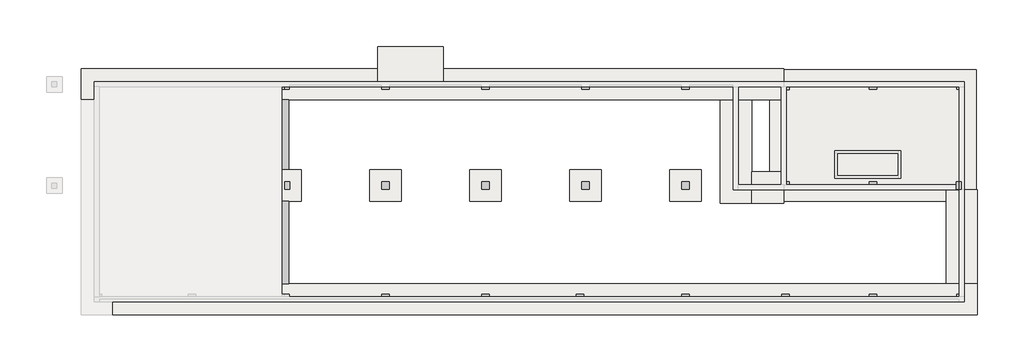
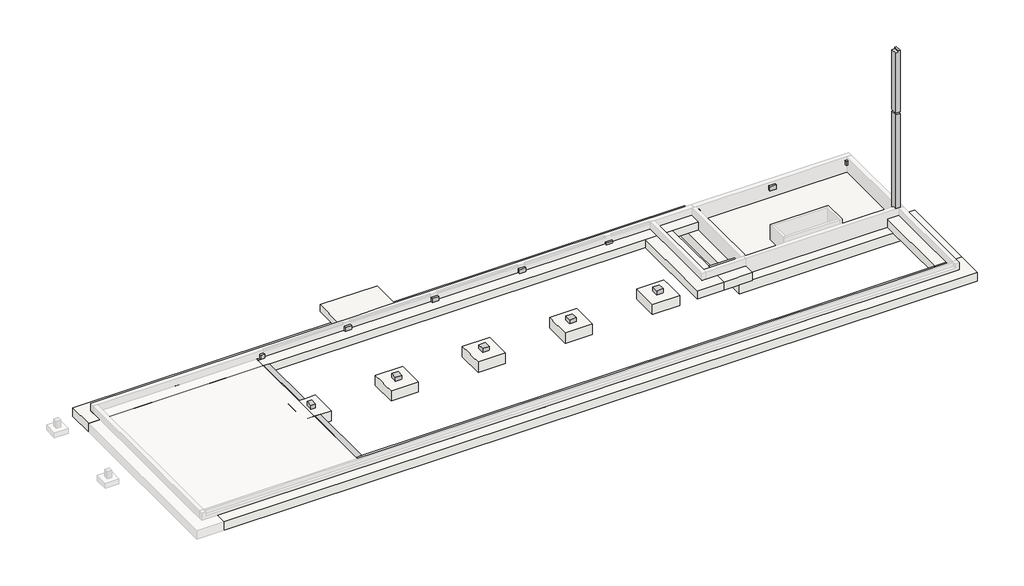
# Not in any storey, part 2 of 2: 25 columns, 8 beams, 8 slabs, 5 footings.
"""IFC4 building model written with IfcOpenShell, lengths in millimetres."""

from ifc_helpers import new_model, si_unit, frame, origin, place, context, project, spatial, polyline, outline, extrude, faceted_brep, element, save

model = new_model("IFC4")

# Units and contexts
model_context = context("Model", 3, world=origin())
ifc_project = project(units=[si_unit("LENGTHUNIT", "METRE", prefix="MILLI")], contexts=[model_context])

# Site, building
site = spatial("IfcSite", under=ifc_project)
building = spatial("IfcBuilding", under=site)

# Beams
placement = place(None, origin())
element("IfcBeam", 1, ObjectType="RC Beam_Rectangular : H_SB_AR_S16_TG_B600xH800_FG2", at=placement, inside=building, context=model_context, shape_type="Brep", body=[
    faceted_brep([(1150.0, 9199.5208589, -1350.0381366), (6250.0, 9199.5208589, -1350.0381366), (6250.0, 9199.5208589, -700.0381366), (4000.0, 9199.5208589, -700.0381366), (3500.0, 9199.5208589, -700.0381366), (1150.0, 9199.5208589, -700.0381366), (1150.0, 9799.5208589, -1350.0381366), (6250.0, 9799.5208589, -1350.0381366), (1150.0, 9799.5208589, -700.0381366), (3500.0, 9799.5208589, -700.0381366), (4000.0, 9799.5208589, -700.0381366), (6250.0, 9799.5208589, -700.0381366)], [[[0, 1, 2, 3, 4, 5]], [[0, 6, 7, 1]], [[7, 6, 8, 9, 10, 11]], [[6, 0, 5, 8]], [[1, 7, 11, 2]], [[5, 4, 3, 2, 11, 10, 9, 8]]]),
])
element("IfcBeam", 2, ObjectType="RC Beam_Rectangular : H_SB_AR_S16_TG_B600xH800_FG2", at=placement, inside=building, context=model_context, shape_type="Brep", body=[
    faceted_brep([(8750.0, 9199.5208589, -1350.0381366), (13750.0, 9199.5208589, -1350.0381366), (13750.0, 9199.5208589, -700.0381366), (11500.0, 9199.5208589, -700.0381366), (11000.0, 9199.5208589, -700.0381366), (8750.0, 9199.5208589, -700.0381366), (8750.0, 9799.5208589, -1350.0381366), (13750.0, 9799.5208589, -1350.0381366), (8750.0, 9799.5208589, -700.0381366), (11000.0, 9799.5208589, -700.0381366), (11500.0, 9799.5208589, -700.0381366), (13750.0, 9799.5208589, -700.0381366)], [[[0, 1, 2, 3, 4, 5]], [[0, 6, 7, 1]], [[7, 6, 8, 9, 10, 11]], [[6, 0, 5, 8]], [[1, 7, 11, 2]], [[5, 4, 3, 2, 11, 10, 9, 8]]]),
])
element("IfcBeam", 3, ObjectType="RC Beam_Rectangular : H_SB_AR_S16_TG_B500xH700_FB1", at=placement, inside=building, context=model_context, shape_type="SweptSolid", body=[
    extrude(outline(polyline([(4000.0, 9799.5208589), (3500.0, 9799.5208589), (3500.0, 16349.5208589), (4000.0, 16349.5208589), (4000.0, 9799.5208589)])), frame((0.0, 0.0, -1250.0381366), z_axis=(0.0, 0.0, 1.0), x_axis=(1.0, 0.0, 0.0)), (0.0, 0.0, 1.0), 550.0),
])
element("IfcBeam", 4, ObjectType="RC Beam_Rectangular : H_SB_AR_S16_TG_B500xH700_FB1", at=placement, inside=building, context=model_context, shape_type="SweptSolid", body=[
    extrude(outline(polyline([(11500.0, 9799.5208589), (11000.0, 9799.5208589), (11000.0, 16349.5208589), (11500.0, 16349.5208589), (11500.0, 9799.5208589)])), frame((0.0, 0.0, -1250.0381366), z_axis=(0.0, 0.0, 1.0), x_axis=(1.0, 0.0, 0.0)), (0.0, 0.0, 1.0), 550.0),
])
element("IfcBeam", 5, ObjectType="RC Beam_Rectangular : H_SB_AR_S16_TG_B500xH700_FB1", at=placement, inside=building, context=model_context, shape_type="SweptSolid", body=[
    extrude(outline(polyline([(11500.0, 1649.5208589), (11000.0, 1649.5208589), (11000.0, 9199.5208589), (11500.0, 9199.5208589), (11500.0, 1649.5208589)])), frame((0.0, 0.0, -1250.0381366), z_axis=(0.0, 0.0, 1.0), x_axis=(1.0, 0.0, 0.0)), (0.0, 0.0, 1.0), 550.0),
])
element("IfcBeam", 6, ObjectType="RC Beam_Rectangular : H_SB_AR_S16_TG_B500xH700_FG1", at=placement, inside=building, context=model_context, shape_type="SweptSolid", body=[
    extrude(outline(polyline([(7250.0, 16349.5208589), (7750.0, 16349.5208589), (7750.0, 10749.5208589), (7250.0, 10749.5208589), (7250.0, 16349.5208589)])), frame((0.0, 0.0, -1250.0381366), z_axis=(0.0, 0.0, 1.0), x_axis=(1.0, 0.0, 0.0)), (0.0, 0.0, 1.0), 550.0),
])
element("IfcBeam", 7, ObjectType="RC Beam_Rectangular : H_SB_AR_S16_TG_B500xH700_FG1", at=placement, inside=building, context=model_context, shape_type="SweptSolid", body=[
    extrude(outline(polyline([(14750.0, 16349.5208589), (15250.0, 16349.5208589), (15250.0, 10749.5208589), (14750.0, 10749.5208589), (14750.0, 16349.5208589)])), frame((0.0, 0.0, -1250.0381366), z_axis=(0.0, 0.0, 1.0), x_axis=(1.0, 0.0, 0.0)), (0.0, 0.0, 1.0), 700.0),
])
element("IfcBeam", 8, ObjectType="RC Beam_Rectangular : H_SB_AR_S16_TG_B500xH700_FG1", at=placement, inside=building, context=model_context, shape_type="SweptSolid", body=[
    extrude(outline(polyline([(15250.0, 1649.5208589), (14750.0, 1649.5208589), (14750.0, 8249.5208589), (15250.0, 8249.5208589), (15250.0, 1649.5208589)])), frame((0.0, 0.0, -1250.0381366), z_axis=(0.0, 0.0, 1.0), x_axis=(1.0, 0.0, 0.0)), (0.0, 0.0, 1.0), 700.0),
])

# Columns
element("IfcColumn", 9, ObjectType="RC_Column_Rectangular : H_SC_AR_S15_UG_W600xL600_C2", at=placement, inside=building, context=model_context, shape_type="Brep", body=[
    faceted_brep([(300.0, 17799.5208589, -850.0381366), (300.0, 17199.5208589, -850.0381366), (-300.0, 17199.5208589, -850.0381366), (-300.0, 17799.5208589, -850.0381366), (300.0, 17799.5208589, -550.0381366), (300.0, 17399.5208589, -550.0381366), (300.0, 17399.5208589, -700.0381366), (300.0, 17199.5208589, -700.0381366), (-300.0, 17199.5208589, -550.0381366), (-300.0, 17399.5208589, -550.0381366), (-300.0, 17799.5208589, -550.0381366), (100.0, 17199.5208589, -550.0381366), (100.0, 17399.5208589, -550.0381366), (100.0, 17399.5208589, -700.0381366), (100.0, 17199.5208589, -700.0381366)], [[[0, 1, 2, 3]], [[1, 0, 4, 5, 6, 7]], [[3, 2, 8, 9, 10]], [[0, 3, 10, 4]], [[8, 11, 12, 5, 4, 10, 9]], [[6, 13, 14, 7]], [[13, 12, 11, 14]], [[12, 13, 6, 5]], [[2, 1, 7, 14, 11, 8]]]),
])
element("IfcColumn", 10, ObjectType="RC_Column_Rectangular : H_SC_AR_S15_UG_W600xL600_C2", at=placement, inside=building, context=model_context, shape_type="SweptSolid", body=[
    extrude(outline(polyline([(17799.5208589, -850.0381366), (17199.5208589, -850.0381366), (17199.5208589, -700.0381366), (17399.5208589, -700.0381366), (17399.5208589, -550.0381366), (17799.5208589, -550.0381366), (17799.5208589, -850.0381366)])), frame((7200.0, 0.0, 0.0), z_axis=(1.0, 0.0, 0.0), x_axis=(0.0, 1.0, 0.0)), (0.0, 0.0, 1.0), 600.0),
])
element("IfcColumn", 11, ObjectType="RC_Column_Rectangular : H_SC_AR_S15_UG_W600xL600_C2", at=placement, inside=building, context=model_context, shape_type="Brep", body=[
    faceted_brep([(15300.0, 17799.5208589, -850.0381366), (15300.0, 17199.5208589, -850.0381366), (14700.0, 17199.5208589, -850.0381366), (14700.0, 17799.5208589, -850.0381366), (15300.0, 17799.5208589, -550.0381366), (15300.0, 17399.5208589, -550.0381366), (15300.0, 17399.5208589, -150.0381366), (15300.0, 17199.5208589, -150.0381366), (14950.0, 17199.5208589, -150.0381366), (14950.0, 17199.5208589, -550.0381366), (14700.0, 17199.5208589, -550.0381366), (14700.0, 17399.5208589, -550.0381366), (14700.0, 17799.5208589, -550.0381366), (14950.0, 17399.5208589, -150.0381366), (14950.0, 17399.5208589, -550.0381366)], [[[0, 1, 2, 3]], [[1, 0, 4, 5, 6, 7]], [[2, 1, 7, 8, 9, 10]], [[3, 2, 10, 11, 12]], [[0, 3, 12, 4]], [[8, 7, 6, 13]], [[14, 9, 8, 13]], [[9, 14, 5, 4, 12, 11, 10]], [[5, 14, 13, 6]]]),
])
element("IfcColumn", 12, ObjectType="RC_Column_Rectangular : H_SC_AR_S15_UG_W600xL600_C2", at=placement, inside=building, context=model_context, shape_type="SweptSolid", body=[
    extrude(outline(polyline([(17799.5208589, -850.0381366), (17199.5208589, -850.0381366), (17199.5208589, -150.0381366), (17399.5208589, -150.0381366), (17399.5208589, -550.0381366), (17799.5208589, -550.0381366), (17799.5208589, -850.0381366)])), frame((22700.0, 0.0, 0.0), z_axis=(1.0, 0.0, 0.0), x_axis=(0.0, 1.0, 0.0)), (0.0, 0.0, 1.0), 600.0),
])
element("IfcColumn", 13, ObjectType="RC_Column_Rectangular : H_SC_AR_S15_UG_W600xL600_C2", at=placement, inside=building, context=model_context, shape_type="SweptSolid", body=[
    extrude(outline(polyline([(17799.5208589, -850.0381366), (17199.5208589, -850.0381366), (17199.5208589, -150.0381366), (17399.5208589, -150.0381366), (17399.5208589, -550.0381366), (17799.5208589, -550.0381366), (17799.5208589, -850.0381366)])), frame((30700.0, 0.0, 0.0), z_axis=(1.0, 0.0, 0.0), x_axis=(0.0, 1.0, 0.0)), (0.0, 0.0, 1.0), 600.0),
])
element("IfcColumn", 14, ObjectType="RC_Column_Rectangular : H_SC_AR_S15_UG_W600xL600_C2", at=placement, inside=building, context=model_context, shape_type="SweptSolid", body=[
    extrude(outline(polyline([(17799.5208589, -850.0381366), (17199.5208589, -850.0381366), (17199.5208589, -150.0381366), (17399.5208589, -150.0381366), (17399.5208589, -550.0381366), (17799.5208589, -550.0381366), (17799.5208589, -850.0381366)])), frame((38700.0, 0.0, 0.0), z_axis=(1.0, 0.0, 0.0), x_axis=(0.0, 1.0, 0.0)), (0.0, 0.0, 1.0), 600.0),
])
element("IfcColumn", 15, ObjectType="RC_Column_Rectangular : H_SC_AR_S15_UG_W600xL600_C2", at=placement, inside=building, context=model_context, shape_type="SweptSolid", body=[
    extrude(outline(polyline([(17799.5208589, -850.0381366), (17199.5208589, -850.0381366), (17199.5208589, -359.953022), (17399.5208589, -359.953022), (17399.5208589, -550.0381366), (17799.5208589, -550.0381366), (17799.5208589, -850.0381366)])), frame((46700.0, 0.0, 0.0), z_axis=(1.0, 0.0, 0.0), x_axis=(0.0, 1.0, 0.0)), (0.0, 0.0, 1.0), 600.0),
])
element("IfcColumn", 16, ObjectType="RC_Column_Rectangular : H_SC_AR_S15_UG_W600xL600_C2", at=placement, inside=building, context=model_context, shape_type="Brep", body=[
    faceted_brep([(69300.0, 799.5208589, -850.0381366), (69300.0, 199.5208589, -850.0381366), (68700.0, 199.5208589, -850.0381366), (68700.0, 799.5208589, -850.0381366), (69300.0, 799.5208589, -550.0381366), (69300.0, 599.5208589, -550.0381366), (69300.0, 199.5208589, -550.0381366), (68700.0, 199.5208589, -550.0381366), (68700.0, 599.5208589, -550.0381366), (68700.0, 599.5208589, -150.0381366), (68700.0, 799.5208589, -150.0381366), (68900.0, 799.5208589, -150.0381366), (68900.0, 799.5208589, -550.0381366), (68900.0, 599.5208589, -150.0381366), (68900.0, 599.5208589, -550.0381366)], [[[0, 1, 2, 3]], [[1, 0, 4, 5, 6]], [[2, 1, 6, 7]], [[3, 2, 7, 8, 9, 10]], [[0, 3, 10, 11, 12, 4]], [[10, 9, 13, 11]], [[9, 8, 14, 13]], [[4, 12, 14, 8, 7, 6, 5]], [[14, 12, 11, 13]]]),
])
element("IfcColumn", 17, ObjectType="RC_Column_Rectangular : H_SC_AR_S15_UG_W600xL600_C2", at=placement, inside=building, context=model_context, shape_type="SweptSolid", body=[
    extrude(outline(polyline([(799.5208589, -850.0381366), (199.5208589, -850.0381366), (199.5208589, -550.0381366), (599.5208589, -550.0381366), (599.5208589, -150.0381366), (799.5208589, -150.0381366), (799.5208589, -850.0381366)])), frame((61700.0, 0.0, 0.0), z_axis=(1.0, 0.0, 0.0), x_axis=(0.0, 1.0, 0.0)), (0.0, 0.0, 1.0), 600.0),
])
element("IfcColumn", 18, ObjectType="RC_Column_Rectangular : H_SC_AR_S15_UG_W600xL600_C2", at=placement, inside=building, context=model_context, shape_type="SweptSolid", body=[
    extrude(outline(polyline([(799.5208589, -850.0381366), (199.5208589, -850.0381366), (199.5208589, -550.0381366), (599.5208589, -550.0381366), (599.5208589, -150.0381366), (799.5208589, -150.0381366), (799.5208589, -850.0381366)])), frame((54700.0, 0.0, 0.0), z_axis=(1.0, 0.0, 0.0), x_axis=(0.0, 1.0, 0.0)), (0.0, 0.0, 1.0), 600.0),
])
element("IfcColumn", 19, ObjectType="RC_Column_Rectangular : H_SC_AR_S15_UG_W600xL600_C2", at=placement, inside=building, context=model_context, shape_type="SweptSolid", body=[
    extrude(outline(polyline([(799.5208589, -850.0381366), (199.5208589, -850.0381366), (199.5208589, -550.0381366), (599.5208589, -550.0381366), (599.5208589, -150.0381366), (799.5208589, -150.0381366), (799.5208589, -850.0381366)])), frame((46700.0, 0.0, 0.0), z_axis=(1.0, 0.0, 0.0), x_axis=(0.0, 1.0, 0.0)), (0.0, 0.0, 1.0), 600.0),
])
element("IfcColumn", 20, ObjectType="RC_Column_Rectangular : H_SC_AR_S15_UG_W600xL600_C2", at=placement, inside=building, context=model_context, shape_type="SweptSolid", body=[
    extrude(outline(polyline([(799.5208589, -850.0381366), (199.5208589, -850.0381366), (199.5208589, -550.0381366), (599.5208589, -550.0381366), (599.5208589, -150.0381366), (799.5208589, -150.0381366), (799.5208589, -850.0381366)])), frame((38250.0, 0.0, 0.0), z_axis=(1.0, 0.0, 0.0), x_axis=(0.0, 1.0, 0.0)), (0.0, 0.0, 1.0), 600.0),
])
element("IfcColumn", 21, ObjectType="RC_Column_Rectangular : H_SC_AR_S15_UG_W600xL600_C2", at=placement, inside=building, context=model_context, shape_type="SweptSolid", body=[
    extrude(outline(polyline([(799.5208589, -850.0381366), (199.5208589, -850.0381366), (199.5208589, -550.0381366), (599.5208589, -550.0381366), (599.5208589, -150.0381366), (799.5208589, -150.0381366), (799.5208589, -850.0381366)])), frame((30700.0, 0.0, 0.0), z_axis=(1.0, 0.0, 0.0), x_axis=(0.0, 1.0, 0.0)), (0.0, 0.0, 1.0), 600.0),
])
element("IfcColumn", 22, ObjectType="RC_Column_Rectangular : H_SC_AR_S15_UG_W600xL600_C2", at=placement, inside=building, context=model_context, shape_type="SweptSolid", body=[
    extrude(outline(polyline([(799.5208589, -850.0381366), (199.5208589, -850.0381366), (199.5208589, -550.0381366), (599.5208589, -550.0381366), (599.5208589, -150.0381366), (799.5208589, -150.0381366), (799.5208589, -850.0381366)])), frame((22700.0, 0.0, 0.0), z_axis=(1.0, 0.0, 0.0), x_axis=(0.0, 1.0, 0.0)), (0.0, 0.0, 1.0), 600.0),
])
element("IfcColumn", 23, ObjectType="RC_Column_Rectangular : H_SC_AR_S15_AG_W600xL600_C2", at=placement, inside=building, context=model_context, shape_type="SweptSolid", body=[
    extrude(outline(polyline([(15350.0, 9799.5208589), (15350.0, 9199.5208589), (14950.0, 9199.5208589), (14950.0, 9799.5208589), (15350.0, 9799.5208589)])), frame((0.0, 0.0, -550.0381366), z_axis=(0.0, 0.0, 1.0), x_axis=(1.0, 0.0, 0.0)), (0.0, 0.0, 1.0), 400.0),
])
element("IfcColumn", 24, ObjectType="RC_Column_Rectangular : H_SC_AR_S15_AG_W600xL600_C2", at=placement, inside=building, context=model_context, shape_type="SweptSolid", body=[
    extrude(outline(polyline([(23300.0, 9799.5208589), (23300.0, 9199.5208589), (22700.0, 9199.5208589), (22700.0, 9799.5208589), (23300.0, 9799.5208589)])), frame((0.0, 0.0, -550.0381366), z_axis=(0.0, 0.0, 1.0), x_axis=(1.0, 0.0, 0.0)), (0.0, 0.0, 1.0), 400.0),
])
element("IfcColumn", 25, ObjectType="RC_Column_Rectangular : H_SC_AR_S15_AG_W600xL600_C2", at=placement, inside=building, context=model_context, shape_type="SweptSolid", body=[
    extrude(outline(polyline([(31300.0, 9799.5208589), (31300.0, 9199.5208589), (30700.0, 9199.5208589), (30700.0, 9799.5208589), (31300.0, 9799.5208589)])), frame((0.0, 0.0, -550.0381366), z_axis=(0.0, 0.0, 1.0), x_axis=(1.0, 0.0, 0.0)), (0.0, 0.0, 1.0), 400.0),
])
element("IfcColumn", 26, ObjectType="RC_Column_Rectangular : H_SC_AR_S15_AG_W600xL600_C2", at=placement, inside=building, context=model_context, shape_type="SweptSolid", body=[
    extrude(outline(polyline([(39300.0, 9799.5208589), (39300.0, 9199.5208589), (38700.0, 9199.5208589), (38700.0, 9799.5208589), (39300.0, 9799.5208589)])), frame((0.0, 0.0, -550.0381366), z_axis=(0.0, 0.0, 1.0), x_axis=(1.0, 0.0, 0.0)), (0.0, 0.0, 1.0), 400.0),
])
element("IfcColumn", 27, ObjectType="RC_Column_Rectangular : H_SC_AR_S15_AG_W600xL600_C2", at=placement, inside=building, context=model_context, shape_type="SweptSolid", body=[
    extrude(outline(polyline([(47300.0, 9799.5208589), (47300.0, 9199.5208589), (46700.0, 9199.5208589), (46700.0, 9799.5208589), (47300.0, 9799.5208589)])), frame((0.0, 0.0, -550.0381366), z_axis=(0.0, 0.0, 1.0), x_axis=(1.0, 0.0, 0.0)), (0.0, 0.0, 1.0), 400.0),
])
element("IfcColumn", 28, ObjectType="RC_Column_Rectangular : H_SC_AR_S15_AG_W600xL600_C2", at=placement, inside=building, context=model_context, shape_type="SweptSolid", body=[
    extrude(outline(polyline([(55300.0, 9799.5208589), (55300.0, 9549.5208589), (55050.0, 9549.5208589), (55050.0, 9799.5208589), (55300.0, 9799.5208589)])), frame((0.0, 0.0, -550.0381366), z_axis=(0.0, 0.0, 1.0), x_axis=(1.0, 0.0, 0.0)), (0.0, 0.0, 1.0), 400.0),
])
element("IfcColumn", 29, ObjectType="RC_Column_Rectangular : H_SC_AR_S15_AG_W600xL600_C2", at=placement, inside=building, context=model_context, shape_type="SweptSolid", body=[
    extrude(outline(polyline([(61700.0, 9799.5208589), (62300.0, 9799.5208589), (62300.0, 9549.5208589), (61700.0, 9549.5208589), (61700.0, 9799.5208589)])), frame((0.0, 0.0, -550.0381366), z_axis=(0.0, 0.0, 1.0), x_axis=(1.0, 0.0, 0.0)), (0.0, 0.0, 1.0), 400.0),
])
element("IfcColumn", 30, ObjectType="RC_Column_Rectangular : H_SC_AR_S15_AG_W600xL600_C2", at=placement, inside=building, context=model_context, shape_type="Brep", body=[
    faceted_brep([(68650.0, 9799.5208589, -550.0381366), (68900.0, 9799.5208589, -550.0381366), (68900.0, 9549.5208589, -550.0381366), (68650.0, 9549.5208589, -550.0381366), (68900.0, 9799.5208589, 149.9618634), (68900.0, 9549.5208589, 149.9618634), (68650.0, 9549.5208589, 149.9618634), (69050.0, 9799.5208589, 149.9618634), (69050.0, 9199.5208589, 149.9618634), (68650.0, 9199.5208589, 149.9618634), (69050.0, 9799.5208589, 9269.9618634), (69050.0, 9199.5208589, 9269.9618634), (68650.0, 9199.5208589, 9269.9618634), (68650.0, 9799.5208589, 9269.9618634)], [[[0, 1, 2, 3]], [[1, 4, 5, 2]], [[6, 5, 4, 7, 8, 9]], [[5, 6, 3, 2]], [[8, 7, 10, 11]], [[12, 11, 10, 13]], [[9, 8, 11, 12]], [[0, 3, 6, 9, 12, 13]], [[1, 0, 13, 10, 7, 4]]]),
    faceted_brep([(69050.0, 9199.5208589, 9449.9618634), (69050.0, 9199.5208589, 15409.9618634), (68900.0, 9199.5208589, 15409.9618634), (68900.0, 9199.5208589, 15259.9618634), (68650.0, 9199.5208589, 15259.9618634), (68650.0, 9199.5208589, 9449.9618634), (68650.0, 9799.5208589, 9449.9618634), (68650.0, 9799.5208589, 15259.9618634), (69050.0, 9799.5208589, 15409.9618634), (69050.0, 9799.5208589, 9449.9618634), (68900.0, 9799.5208589, 15259.9618634), (68900.0, 9799.5208589, 15409.9618634)], [[[0, 1, 2, 3, 4, 5]], [[6, 5, 4, 7]], [[8, 9, 6, 7, 10, 11]], [[1, 8, 11, 2]], [[0, 5, 6, 9]], [[8, 1, 0, 9]], [[3, 10, 7, 4]], [[10, 3, 2, 11]]]),
])
element("IfcColumn", 31, ObjectType="RC_Column_Rectangular : H_SC_AR_S15_UG_W600xL600_C2", at=placement, inside=building, context=model_context, shape_type="SweptSolid", body=[
    extrude(outline(polyline([(68700.0, 17199.5208589), (68700.0, 17399.5208589), (68900.0, 17399.5208589), (68900.0, 17199.5208589), (68700.0, 17199.5208589)])), frame((0.0, 0.0, -550.0381366), z_axis=(0.0, 0.0, 1.0), x_axis=(1.0, 0.0, 0.0)), (0.0, 0.0, 1.0), 400.0),
])
element("IfcColumn", 32, ObjectType="RC_Column_Rectangular : H_SC_AR_S15_UG_W600xL600_C2", at=placement, inside=building, context=model_context, shape_type="SweptSolid", body=[
    extrude(outline(polyline([(62300.0, 17199.5208589), (61700.0, 17199.5208589), (61700.0, 17399.5208589), (62300.0, 17399.5208589), (62300.0, 17199.5208589)])), frame((0.0, 0.0, -550.0381366), z_axis=(0.0, 0.0, 1.0), x_axis=(1.0, 0.0, 0.0)), (0.0, 0.0, 1.0), 400.0),
])
element("IfcColumn", 33, ObjectType="RC_Column_Rectangular : H_SC_AR_S15_AG_W600xL600_C2", at=placement, inside=building, context=model_context, shape_type="SweptSolid", body=[
    extrude(outline(polyline([(54850.0, 17749.5208589), (54850.0, 17399.5208589), (54700.0, 17399.5208589), (54700.0, 17749.5208589), (54850.0, 17749.5208589)])), frame((0.0, 0.0, -550.0381366), z_axis=(0.0, 0.0, 1.0), x_axis=(1.0, 0.0, 0.0)), (0.0, 0.0, 1.0), 400.0),
    extrude(outline(polyline([(55300.0, 17399.5208589), (55300.0, 17149.5208589), (55050.0, 17149.5208589), (55050.0, 17399.5208589), (55300.0, 17399.5208589)])), frame((0.0, 0.0, -550.0381366), z_axis=(0.0, 0.0, 1.0), x_axis=(1.0, 0.0, 0.0)), (0.0, 0.0, 1.0), 400.0),
])

# Footings
element("IfcFooting", 34, ObjectType="H_SF_AR_S18_Wall FDN_T800", at=placement, inside=building, context=model_context, shape_type="Brep", body=[
    faceted_brep([(54850.0, 18849.5208589, -550.0381366), (54850.0, 16349.5208589, -550.0381366), (54850.0, 16349.5208589, -1350.0381366), (54850.0, 18849.5208589, -1350.0381366), (-1350.0, 16349.5208589, -550.0381366), (1150.0, 16349.5208589, -550.0381366), (14750.0, 16349.5208589, -550.0381366), (15250.0, 16349.5208589, -550.0381366), (49775.0, 16349.5208589, -550.0381366), (52275.0, 16349.5208589, -550.0381366), (-1350.0, 18849.5208589, -550.0381366), (-1350.0, 18849.5208589, -1350.0381366), (-1350.0, 16349.5208589, -1350.0381366), (52275.0, 16349.5208589, -1350.0381366), (49775.0, 16349.5208589, -1350.0381366), (1150.0, 16349.5208589, -1350.0381366)], [[[0, 1, 2, 3]], [[4, 5, 6, 7, 8, 9, 1, 0, 10]], [[11, 10, 0, 3]], [[12, 11, 3, 2, 13, 14, 15]], [[4, 12, 15, 14, 13, 2, 1, 9, 8, 7, 6, 5]], [[4, 10, 11, 12]]]),
])
element("IfcFooting", 35, ObjectType="H_SF_AR_S18_Wall FDN_T800", at=placement, inside=building, context=model_context, shape_type="Brep", body=[
    faceted_brep([(70350.0, -850.4791411, -550.0381366), (70350.0, 1649.5208589, -550.0381366), (67850.0, 1649.5208589, -550.0381366), (15250.0, 1649.5208589, -550.0381366), (14750.0, 1649.5208589, -550.0381366), (1150.0, 1649.5208589, -550.0381366), (1150.0, -850.4791411, -550.0381366), (70350.0, -850.4791411, -1350.0381366), (1150.0, -850.4791411, -1350.0381366), (70350.0, 1649.5208589, -1350.0381366), (1150.0, 1649.5208589, -1350.0381366), (67850.0, 1649.5208589, -1350.0381366)], [[[0, 1, 2, 3, 4, 5, 6]], [[7, 0, 6, 8]], [[9, 7, 8, 10, 11]], [[1, 9, 11, 10, 5, 4, 3, 2]], [[1, 0, 7, 9]], [[6, 5, 10, 8]]]),
])
element("IfcFooting", 36, ObjectType="H_SF_AR_S18_Wall FDN_T800", at=placement, inside=building, context=model_context, shape_type="SweptSolid", body=[
    extrude(outline(polyline([(67850.0, 9149.5208589), (70350.0, 9149.5208589), (70350.0, 1649.5208589), (67850.0, 1649.5208589), (67850.0, 9149.5208589)])), frame((0.0, 0.0, -1350.0381366), z_axis=(0.0, 0.0, 1.0), x_axis=(1.0, 0.0, 0.0)), (0.0, 0.0, 1.0), 800.0),
])
element("IfcFooting", 37, ObjectType="H_SF_AR_S18_Wall FDN_T800", at=placement, inside=building, context=model_context, shape_type="Brep", body=[
    faceted_brep([(49775.0, 16349.5208589, -550.0381366), (49775.0, 9799.5208589, -550.0381366), (49775.0, 9199.5208589, -550.0381366), (49775.0, 8099.5208589, -550.0381366), (52275.0, 8099.5208589, -550.0381366), (52275.0, 10599.5208589, -550.0381366), (52275.0, 16349.5208589, -550.0381366), (52275.0, 16349.5208589, -1350.0381366), (52275.0, 8099.5208589, -1350.0381366), (52275.0, 10599.5208589, -1350.0381366), (49775.0, 16349.5208589, -1350.0381366), (49775.0, 8099.5208589, -1350.0381366)], [[[0, 1, 2, 3, 4, 5, 6]], [[7, 6, 5, 4, 8, 9]], [[10, 7, 9, 8, 11]], [[0, 10, 11, 3, 2, 1]], [[0, 6, 7, 10]], [[4, 3, 11, 8]]]),
])
element("IfcFooting", 38, ObjectType="H_SF_AR_S18_Wall FDN_T800", at=placement, inside=building, context=model_context, shape_type="SweptSolid", body=[
    extrude(outline(polyline([(54850.0, 10599.5208589), (54850.0, 8099.5208589), (52275.0, 8099.5208589), (52275.0, 10599.5208589), (54850.0, 10599.5208589)])), frame((0.0, 0.0, -1350.0381366), z_axis=(0.0, 0.0, 1.0), x_axis=(1.0, 0.0, 0.0)), (0.0, 0.0, 1.0), 800.0),
])

# Slabs
element("IfcSlab", 39, ObjectType="H_SF_AR_B01_MAT_Bitumen_MF1", at=placement, inside=building, context=model_context, shape_type="SweptSolid", body=[
    extrude(outline(polyline([(70250.0, 18749.5208589), (70250.0, 8249.5208589), (53750.0, 8249.5208589), (53750.0, 18749.5208589), (70250.0, 18749.5208589)])), frame((0.0, 0.0, -2350.0381366), z_axis=(0.0, 0.0, 1.0), x_axis=(1.0, 0.0, 0.0)), (0.0, 0.0, 1.0), 1000.0),
])
element("IfcSlab", 40, ObjectType="H_SF_AR_B01_MAT_Bitumen_MF2", at=placement, inside=building, context=model_context, shape_type="Brep", body=[
    faceted_brep([(27625.0, 20624.5208589, -550.0381366), (27625.0, 17799.5208589, -550.0381366), (22375.0, 17799.5208589, -550.0381366), (22375.0, 20624.5208589, -550.0381366), (27625.0, 20624.5208589, 99.9618634), (22375.0, 20624.5208589, 99.9618634), (22375.0, 17799.5208589, 99.9618634), (27625.0, 17799.5208589, 99.9618634), (22375.0, 17799.5208589, -50.0381366)], [[[0, 1, 2, 3]], [[4, 5, 6, 7]], [[1, 0, 4, 7]], [[2, 1, 7, 6, 8]], [[3, 2, 8, 6, 5]], [[0, 3, 5, 4]]]),
])
element("IfcSlab", 41, ObjectType="Foundation Rectangular (Non-Pile) : H_SF_AR_S18_W2500xL2500xT1000_Bitumen_F1", at=placement, inside=building, context=model_context, shape_type="Brep", body=[
    faceted_brep([(8750.0, 10749.5208589, -1550.0381366), (8750.0, 8249.5208589, -1550.0381366), (6250.0, 8249.5208589, -1550.0381366), (6250.0, 10749.5208589, -1550.0381366), (6250.0, 10749.5208589, -700.0381366), (7250.0, 10749.5208589, -700.0381366), (7750.0, 10749.5208589, -700.0381366), (8750.0, 10749.5208589, -700.0381366), (6250.0, 8249.5208589, -700.0381366), (6250.0, 9199.5208589, -700.0381366), (6250.0, 9799.5208589, -700.0381366), (8750.0, 8249.5208589, -700.0381366), (7750.0, 8249.5208589, -700.0381366), (7250.0, 8249.5208589, -700.0381366), (8750.0, 9799.5208589, -700.0381366), (8750.0, 9199.5208589, -700.0381366)], [[[0, 1, 2, 3]], [[0, 3, 4, 5, 6, 7]], [[3, 2, 8, 9, 10, 4]], [[2, 1, 11, 12, 13, 8]], [[1, 0, 7, 14, 15, 11]], [[7, 6, 5, 4, 10, 9, 8, 13, 12, 11, 15, 14]]]),
])
element("IfcSlab", 42, ObjectType="Foundation Rectangular (Non-Pile) : H_SF_AR_S18_W2500xL2500xT1000_Bitumen_F1", at=placement, inside=building, context=model_context, shape_type="Brep", body=[
    faceted_brep([(16250.0, 10749.5208589, -550.0381366), (15250.0, 10749.5208589, -550.0381366), (14750.0, 10749.5208589, -550.0381366), (13750.0, 10749.5208589, -550.0381366), (13750.0, 8249.5208589, -550.0381366), (14750.0, 8249.5208589, -550.0381366), (15250.0, 8249.5208589, -550.0381366), (16250.0, 8249.5208589, -550.0381366), (16250.0, 9149.5208589, -550.0381366), (16250.0, 9749.5208589, -550.0381366), (16250.0, 10749.5208589, -1550.0381366), (16250.0, 8249.5208589, -1550.0381366), (13750.0, 8249.5208589, -1550.0381366), (13750.0, 10749.5208589, -1550.0381366)], [[[0, 1, 2, 3, 4, 5, 6, 7, 8, 9]], [[10, 11, 12, 13]], [[3, 2, 1, 0, 10, 13]], [[4, 3, 13, 12]], [[7, 6, 5, 4, 12, 11]], [[0, 9, 8, 7, 11, 10]]]),
])
element("IfcSlab", 43, ObjectType="Foundation Rectangular (Non-Pile) : H_SF_AR_S18_W2500xL2500xT1000_Bitumen_F1", at=placement, inside=building, context=model_context, shape_type="Brep", body=[
    faceted_brep([(24250.0, 10749.5208589, -550.0381366), (21750.0, 10749.5208589, -550.0381366), (21750.0, 9749.5208589, -550.0381366), (21750.0, 9149.5208589, -550.0381366), (21750.0, 8249.5208589, -550.0381366), (24250.0, 8249.5208589, -550.0381366), (24250.0, 9149.5208589, -550.0381366), (24250.0, 9749.5208589, -550.0381366), (24250.0, 10749.5208589, -1550.0381366), (24250.0, 8249.5208589, -1550.0381366), (21750.0, 8249.5208589, -1550.0381366), (21750.0, 10749.5208589, -1550.0381366)], [[[0, 1, 2, 3, 4, 5, 6, 7]], [[8, 9, 10, 11]], [[1, 0, 8, 11]], [[4, 3, 2, 1, 11, 10]], [[5, 4, 10, 9]], [[0, 7, 6, 5, 9, 8]]]),
])
element("IfcSlab", 44, ObjectType="Foundation Rectangular (Non-Pile) : H_SF_AR_S18_W2500xL2500xT1000_Bitumen_F1", at=placement, inside=building, context=model_context, shape_type="Brep", body=[
    faceted_brep([(32250.0, 10749.5208589, -550.0381366), (29750.0, 10749.5208589, -550.0381366), (29750.0, 9749.5208589, -550.0381366), (29750.0, 9149.5208589, -550.0381366), (29750.0, 8249.5208589, -550.0381366), (32250.0, 8249.5208589, -550.0381366), (32250.0, 9149.5208589, -550.0381366), (32250.0, 9749.5208589, -550.0381366), (32250.0, 10749.5208589, -1550.0381366), (32250.0, 8249.5208589, -1550.0381366), (29750.0, 8249.5208589, -1550.0381366), (29750.0, 10749.5208589, -1550.0381366)], [[[0, 1, 2, 3, 4, 5, 6, 7]], [[8, 9, 10, 11]], [[1, 0, 8, 11]], [[4, 3, 2, 1, 11, 10]], [[5, 4, 10, 9]], [[0, 7, 6, 5, 9, 8]]]),
])
element("IfcSlab", 45, ObjectType="Foundation Rectangular (Non-Pile) : H_SF_AR_S18_W2500xL2500xT1000_Bitumen_F1", at=placement, inside=building, context=model_context, shape_type="Brep", body=[
    faceted_brep([(40250.0, 10749.5208589, -550.0381366), (37750.0, 10749.5208589, -550.0381366), (37750.0, 9749.5208589, -550.0381366), (37750.0, 9149.5208589, -550.0381366), (37750.0, 8249.5208589, -550.0381366), (40250.0, 8249.5208589, -550.0381366), (40250.0, 9149.5208589, -550.0381366), (40250.0, 9749.5208589, -550.0381366), (40250.0, 10749.5208589, -1550.0381366), (40250.0, 8249.5208589, -1550.0381366), (37750.0, 8249.5208589, -1550.0381366), (37750.0, 10749.5208589, -1550.0381366)], [[[0, 1, 2, 3, 4, 5, 6, 7]], [[8, 9, 10, 11]], [[1, 0, 8, 11]], [[4, 3, 2, 1, 11, 10]], [[5, 4, 10, 9]], [[0, 7, 6, 5, 9, 8]]]),
])
element("IfcSlab", 46, ObjectType="Foundation Rectangular (Non-Pile) : H_SF_AR_S18_W2500xL2500xT1000_Bitumen_F1", at=placement, inside=building, context=model_context, shape_type="Brep", body=[
    faceted_brep([(48250.0, 10749.5208589, -550.0381366), (45750.0, 10749.5208589, -550.0381366), (45750.0, 9749.5208589, -550.0381366), (45750.0, 9149.5208589, -550.0381366), (45750.0, 8249.5208589, -550.0381366), (48250.0, 8249.5208589, -550.0381366), (48250.0, 9199.5208589, -550.0381366), (48250.0, 9799.5208589, -550.0381366), (48250.0, 10749.5208589, -1550.0381366), (48250.0, 8249.5208589, -1550.0381366), (45750.0, 8249.5208589, -1550.0381366), (45750.0, 10749.5208589, -1550.0381366)], [[[0, 1, 2, 3, 4, 5, 6, 7]], [[8, 9, 10, 11]], [[1, 0, 8, 11]], [[4, 3, 2, 1, 11, 10]], [[5, 4, 10, 9]], [[0, 7, 6, 5, 9, 8]]]),
])

save(model, "model.ifc")

# Revit data of these elements
# Type "RC Beam_Rectangular : H_SB_AR_S16_TG_B600xH800_FG2"
#   Type Comments = "CV-UG"
#   Type Mark = "FG2"
#   H_Q'ty Cal Type Tag = "SB-Q1A"
#   H_WM Code_1 = "A03AF032-00022 |  | M3 | Concrete Work | Superstructure Work | Structural Concrete | Cement Type-1 | 25MPa ≤ F'c (Cylinder Strength) < 30MPa |  |  |  |  | A03AF032-00022 Concrete Work Superstructure Work Structural Concrete  Cement Type-1 25MPa ≤ F'c (Cylinder Strength) < 30MPa      |  F'c (Cylinder Strength) = 24MPa"
#   H_WM Code_2 = "A03AD037-00002 |  | TON | Concrete Work | Substructure Work | Rebar Work | Deformed Bar (Non-Coat.) | 400MPa<Fy≤470MPa |  |  |  |  | A03AD037-00002 Concrete Work Substructure Work Rebar Work Deformed Bar (Non-Coat.)  400MPa<Fy≤470MPa      | ASTM A615 GRADE 60 (Fy=420MPa)"
#   H_WM Code_3 = "A03AD035-00001 |  | M2 | Concrete Work | Substructure Work | Form Work (3 times in use) | Flat Form | Dressed Lumber, Plywood or Steel Form(Wood Planks are not Allowed) incl. Chamfer |  |  |  | A03AD035-00001 Concrete Work Substructure Work Form Work (3 times in use) Flat Form     Dressed Lumber, Plywood or Steel Form(Wood Planks are not Allowed) incl. Chamfer   | Dressed Lumber, Plywood or Steel Form(Wood Planks are not Allowed) incl. Chamfer"
#   H_WM Code_4 = "A03AH056-00001 |  | M2 | Concrete Work | Concrete Protective Coating (U/G) | Bitumen/Bituminous/Asphalt Coating |  |  | A03AH056-00001 Concrete Work Concrete Protective Coating (U/G) Bitumen/Bituminous/Asphalt Coating         | Bitumen/Bituminous/Asphalt Coating"
#   H_WM Code_5 = "A03AD047-00004 |  | M2 | Concrete Work | Substructure Work | Insulation under Ground Floor | Extruded Polystyrene Insulation Board |  | 100mm≤THK | THK=(  )mm |  | A03AD047-00004 Concrete Work Substructure Work Insulation under Ground Floor Extruded Polystyrene Insulation Board       100mm≤THK | Bitumen/Bituminous/Asphalt Coating"
#   H_WM Code_6 = "A01ZZ001-00012 |  | M3 | Earth Work | - | Excavation | Soil, Mech. |  | Manual Excavation Above GWL |  |  |  | A01ZZ001-00012 Earth Work - Excavation Soil, Mech.      Manual Excavation Above GWL  | Above GWL"
#   H_WM Code_7 = "A01ZZ001-00013 |  | M3 | Earth Work | - | Excavation | Soil, Mech. |  | Manual Excavation Below GWL |  |  |  | A01ZZ001-00013 Earth Work - Excavation Soil, Mech.      Manual Excavation Below GWL  | Below GWL"
#   H_WM Code_8 = "A01ZZ003-00001 |  | M3 | Earth Work | - | Backfill | Re-use, Soil |  |  |  | Compaction=(  )% |  | A01ZZ003-00001 Earth Work - Backfill Re-use, Soil        | Compaction=( 95 )%"
#   H_WM Code_9 = "A01ZZ004-00001 |  | M3 | Earth Work | - | Disposal | Soil |  |  |  | Disposal Distance=Appx. (  )km from Site |  | A01ZZ004-00001 Earth Work - Disposal Soil        | Disposal Distance=Appx. (20 )km from Site"
#   H_WM Code_10 = "A03AH056-00001 |  | M2 | Concrete Work | Concrete Protective Coating (U/G) | Bitumen/Bituminous/Asphalt Coating |  |  | A03AH056-00001 Concrete Work Concrete Protective Coating (U/G) Bitumen/Bituminous/Asphalt Coating         | *기초바닥 Protection 은 Lean에 적용"
#   중앙부 하부근 = ""
#   중앙부 상부근 = ""
#   중앙부 보조근 = ""
#   중앙부 늑근 = ""
#   외단부 하부근 = ""
#   외단부 상부근 = ""
#   외단부 보조근 = ""
#   외단부 늑근 = ""
#   부호 = "TG2"
#   내단부 하부근 = ""
#   내단부 상부근 = ""
#   내단부 보조근 = ""
#   내단부 늑근 = ""
#   ALL 하부근 = "3-D20"
#   ALL 상부근 = "4-D20"
#   ALL 보조근 = ""
#   ALL 늑근 = "2-D10 @120"
#   H_Rebar ratio = 0.14
#   Width = 600 mm
#   Height = 800 mm
#   Length [instance default] = 1524 mm
#   b = 600 mm
#   h = 800 mm
#   hec_material3 [instance default] = none
#   hec_material2 [instance default] = none
#   hec_material1 [instance default] = none
#   Structural Material [instance default] = none
#   Assembly Code = ""
# Type "RC Beam_Rectangular : H_SB_AR_S16_TG_B500xH700_FB1"
#   Type Comments = "CV-UG"
#   Type Mark = "FB1"
#   H_Q'ty Cal Type Tag = "SB-Q1A"
#   H_WM Code_1 = "A03AF032-00022 |  | M3 | Concrete Work | Superstructure Work | Structural Concrete | Cement Type-1 | 25MPa ≤ F'c (Cylinder Strength) < 30MPa |  |  |  |  | A03AF032-00022 Concrete Work Superstructure Work Structural Concrete  Cement Type-1 25MPa ≤ F'c (Cylinder Strength) < 30MPa      |  F'c (Cylinder Strength) = 24MPa"
#   H_WM Code_2 = "A03AD037-00002 |  | TON | Concrete Work | Substructure Work | Rebar Work | Deformed Bar (Non-Coat.) | 400MPa<Fy≤470MPa |  |  |  |  | A03AD037-00002 Concrete Work Substructure Work Rebar Work Deformed Bar (Non-Coat.)  400MPa<Fy≤470MPa      | ASTM A615 GRADE 60 (Fy=420MPa)"
#   H_WM Code_3 = "A03AD035-00001 |  | M2 | Concrete Work | Substructure Work | Form Work (3 times in use) | Flat Form | Dressed Lumber, Plywood or Steel Form(Wood Planks are not Allowed) incl. Chamfer |  |  |  | A03AD035-00001 Concrete Work Substructure Work Form Work (3 times in use) Flat Form     Dressed Lumber, Plywood or Steel Form(Wood Planks are not Allowed) incl. Chamfer   | Dressed Lumber, Plywood or Steel Form(Wood Planks are not Allowed) incl. Chamfer"
#   H_WM Code_4 = "A03AH056-00001 |  | M2 | Concrete Work | Concrete Protective Coating (U/G) | Bitumen/Bituminous/Asphalt Coating |  |  | A03AH056-00001 Concrete Work Concrete Protective Coating (U/G) Bitumen/Bituminous/Asphalt Coating         | Bitumen/Bituminous/Asphalt Coating"
#   H_WM Code_5 = "A03AD047-00004 |  | M2 | Concrete Work | Substructure Work | Insulation under Ground Floor | Extruded Polystyrene Insulation Board |  | 100mm≤THK | THK=(  )mm |  | A03AD047-00004 Concrete Work Substructure Work Insulation under Ground Floor Extruded Polystyrene Insulation Board       100mm≤THK | Bitumen/Bituminous/Asphalt Coating"
#   H_WM Code_6 = "A01ZZ001-00012 |  | M3 | Earth Work | - | Excavation | Soil, Mech. |  | Manual Excavation Above GWL |  |  |  | A01ZZ001-00012 Earth Work - Excavation Soil, Mech.      Manual Excavation Above GWL  | Above GWL"
#   H_WM Code_7 = "A01ZZ001-00013 |  | M3 | Earth Work | - | Excavation | Soil, Mech. |  | Manual Excavation Below GWL |  |  |  | A01ZZ001-00013 Earth Work - Excavation Soil, Mech.      Manual Excavation Below GWL  | Below GWL"
#   H_WM Code_8 = "A01ZZ003-00001 |  | M3 | Earth Work | - | Backfill | Re-use, Soil |  |  |  | Compaction=(  )% |  | A01ZZ003-00001 Earth Work - Backfill Re-use, Soil        | Compaction=( 95 )%"
#   H_WM Code_9 = "A01ZZ004-00001 |  | M3 | Earth Work | - | Disposal | Soil |  |  |  | Disposal Distance=Appx. (  )km from Site |  | A01ZZ004-00001 Earth Work - Disposal Soil        | Disposal Distance=Appx. (20 )km from Site"
#   H_WM Code_10 = "A03AH056-00001 |  | M2 | Concrete Work | Concrete Protective Coating (U/G) | Bitumen/Bituminous/Asphalt Coating |  |  | A03AH056-00001 Concrete Work Concrete Protective Coating (U/G) Bitumen/Bituminous/Asphalt Coating         | *기초바닥 Protection 은 Lean에 적용"
#   중앙부 하부근 = ""
#   중앙부 상부근 = ""
#   중앙부 보조근 = ""
#   중앙부 늑근 = ""
#   외단부 하부근 = ""
#   외단부 상부근 = ""
#   외단부 보조근 = ""
#   외단부 늑근 = ""
#   부호 = "TG2"
#   내단부 하부근 = ""
#   내단부 상부근 = ""
#   내단부 보조근 = ""
#   내단부 늑근 = ""
#   ALL 하부근 = "3-D20"
#   ALL 상부근 = "4-D20"
#   ALL 보조근 = ""
#   ALL 늑근 = "2-D10 @120"
#   H_Rebar ratio = 0.14
#   Width = 500 mm
#   Height = 700 mm
#   Length [instance default] = 1524 mm
#   b = 500 mm
#   h = 700 mm
#   hec_material3 [instance default] = none
#   hec_material2 [instance default] = none
#   hec_material1 [instance default] = none
#   Structural Material [instance default] = none
#   Assembly Code = ""
# Type "RC Beam_Rectangular : H_SB_AR_S16_TG_B500xH700_FG1"
#   Type Comments = "CV-UG"
#   Type Mark = "FG1"
#   H_Q'ty Cal Type Tag = "SB-Q1A"
#   H_WM Code_1 = "A03AF032-00022 |  | M3 | Concrete Work | Superstructure Work | Structural Concrete | Cement Type-1 | 25MPa ≤ F'c (Cylinder Strength) < 30MPa |  |  |  |  | A03AF032-00022 Concrete Work Superstructure Work Structural Concrete  Cement Type-1 25MPa ≤ F'c (Cylinder Strength) < 30MPa      |  F'c (Cylinder Strength) = 24MPa"
#   H_WM Code_2 = "A03AD037-00002 |  | TON | Concrete Work | Substructure Work | Rebar Work | Deformed Bar (Non-Coat.) | 400MPa<Fy≤470MPa |  |  |  |  | A03AD037-00002 Concrete Work Substructure Work Rebar Work Deformed Bar (Non-Coat.)  400MPa<Fy≤470MPa      | ASTM A615 GRADE 60 (Fy=420MPa)"
#   H_WM Code_3 = "A03AD035-00001 |  | M2 | Concrete Work | Substructure Work | Form Work (3 times in use) | Flat Form | Dressed Lumber, Plywood or Steel Form(Wood Planks are not Allowed) incl. Chamfer |  |  |  | A03AD035-00001 Concrete Work Substructure Work Form Work (3 times in use) Flat Form     Dressed Lumber, Plywood or Steel Form(Wood Planks are not Allowed) incl. Chamfer   | Dressed Lumber, Plywood or Steel Form(Wood Planks are not Allowed) incl. Chamfer"
#   H_WM Code_4 = "A03AH056-00001 |  | M2 | Concrete Work | Concrete Protective Coating (U/G) | Bitumen/Bituminous/Asphalt Coating |  |  | A03AH056-00001 Concrete Work Concrete Protective Coating (U/G) Bitumen/Bituminous/Asphalt Coating         | Bitumen/Bituminous/Asphalt Coating"
#   H_WM Code_5 = "A03AD047-00004 |  | M2 | Concrete Work | Substructure Work | Insulation under Ground Floor | Extruded Polystyrene Insulation Board |  | 100mm≤THK | THK=(  )mm |  | A03AD047-00004 Concrete Work Substructure Work Insulation under Ground Floor Extruded Polystyrene Insulation Board       100mm≤THK | Bitumen/Bituminous/Asphalt Coating"
#   H_WM Code_6 = "A01ZZ001-00012 |  | M3 | Earth Work | - | Excavation | Soil, Mech. |  | Manual Excavation Above GWL |  |  |  | A01ZZ001-00012 Earth Work - Excavation Soil, Mech.      Manual Excavation Above GWL  | Above GWL"
#   H_WM Code_7 = "A01ZZ001-00013 |  | M3 | Earth Work | - | Excavation | Soil, Mech. |  | Manual Excavation Below GWL |  |  |  | A01ZZ001-00013 Earth Work - Excavation Soil, Mech.      Manual Excavation Below GWL  | Below GWL"
#   H_WM Code_8 = "A01ZZ003-00001 |  | M3 | Earth Work | - | Backfill | Re-use, Soil |  |  |  | Compaction=(  )% |  | A01ZZ003-00001 Earth Work - Backfill Re-use, Soil        | Compaction=( 95 )%"
#   H_WM Code_9 = "A01ZZ004-00001 |  | M3 | Earth Work | - | Disposal | Soil |  |  |  | Disposal Distance=Appx. (  )km from Site |  | A01ZZ004-00001 Earth Work - Disposal Soil        | Disposal Distance=Appx. (20 )km from Site"
#   H_WM Code_10 = "A03AH056-00001 |  | M2 | Concrete Work | Concrete Protective Coating (U/G) | Bitumen/Bituminous/Asphalt Coating |  |  | A03AH056-00001 Concrete Work Concrete Protective Coating (U/G) Bitumen/Bituminous/Asphalt Coating         | *기초바닥 Protection 은 Lean에 적용"
#   중앙부 하부근 = ""
#   중앙부 상부근 = ""
#   중앙부 보조근 = ""
#   중앙부 늑근 = ""
#   외단부 하부근 = ""
#   외단부 상부근 = ""
#   외단부 보조근 = ""
#   외단부 늑근 = ""
#   부호 = "TG2"
#   내단부 하부근 = ""
#   내단부 상부근 = ""
#   내단부 보조근 = ""
#   내단부 늑근 = ""
#   ALL 하부근 = "3-D20"
#   ALL 상부근 = "4-D20"
#   ALL 보조근 = ""
#   ALL 늑근 = "2-D10 @120"
#   H_Rebar ratio = 0.14
#   Width = 500 mm
#   Height = 700 mm
#   Length [instance default] = 1524 mm
#   b = 500 mm
#   h = 700 mm
#   hec_material3 [instance default] = none
#   hec_material2 [instance default] = none
#   hec_material1 [instance default] = none
#   Structural Material [instance default] = none
#   Assembly Code = ""
# Type "RC_Column_Rectangular : H_SC_AR_S15_UG_W600xL600_C2"
#   Type Comments = "CV-UG"
#   Type Mark = "C2"
#   H_Q'ty Cal Type Tag = "SB-Q1A"
#   H_WM Code_1 = "A03AF032-00022 |  | M3 | Concrete Work | Superstructure Work | Structural Concrete | Cement Type-1 | 25MPa ≤ F'c (Cylinder Strength) < 30MPa |  |  |  |  | A03AF032-00022 Concrete Work Superstructure Work Structural Concrete  Cement Type-1 25MPa ≤ F'c (Cylinder Strength) < 30MPa      |  F'c (Cylinder Strength) = 24MPa"
#   H_WM Code_2 = "A03AD037-00002 |  | TON | Concrete Work | Substructure Work | Rebar Work | Deformed Bar (Non-Coat.) | 400MPa<Fy≤470MPa |  |  |  |  | A03AD037-00002 Concrete Work Substructure Work Rebar Work Deformed Bar (Non-Coat.)  400MPa<Fy≤470MPa      | ASTM A615 GRADE 60 (Fy=420MPa)"
#   H_WM Code_3 = "A03AD035-00001 |  | M2 | Concrete Work | Substructure Work | Form Work (3 times in use) | Flat Form | Dressed Lumber, Plywood or Steel Form(Wood Planks are not Allowed) incl. Chamfer |  |  |  | A03AD035-00001 Concrete Work Substructure Work Form Work (3 times in use) Flat Form     Dressed Lumber, Plywood or Steel Form(Wood Planks are not Allowed) incl. Chamfer   | Dressed Lumber, Plywood or Steel Form(Wood Planks are not Allowed) incl. Chamfer"
#   H_WM Code_4 = "A03AH056-00001 |  | M2 | Concrete Work | Concrete Protective Coating (U/G) | Bitumen/Bituminous/Asphalt Coating |  |  | A03AH056-00001 Concrete Work Concrete Protective Coating (U/G) Bitumen/Bituminous/Asphalt Coating         | Bitumen/Bituminous/Asphalt Coating"
#   H_WM Code_5 = "A03AD047-00004 |  | M2 | Concrete Work | Substructure Work | Insulation under Ground Floor | Extruded Polystyrene Insulation Board |  | 100mm≤THK | THK=(  )mm |  | A03AD047-00004 Concrete Work Substructure Work Insulation under Ground Floor Extruded Polystyrene Insulation Board       100mm≤THK | Bitumen/Bituminous/Asphalt Coating"
#   H_WM Code_6 = "A01ZZ001-00012 |  | M3 | Earth Work | - | Excavation | Soil, Mech. |  | Manual Excavation Above GWL |  |  |  | A01ZZ001-00012 Earth Work - Excavation Soil, Mech.      Manual Excavation Above GWL  | Above GWL"
#   H_WM Code_7 = "A01ZZ001-00013 |  | M3 | Earth Work | - | Excavation | Soil, Mech. |  | Manual Excavation Below GWL |  |  |  | A01ZZ001-00013 Earth Work - Excavation Soil, Mech.      Manual Excavation Below GWL  | Below GWL"
#   H_WM Code_8 = "A01ZZ003-00001 |  | M3 | Earth Work | - | Backfill | Re-use, Soil |  |  |  | Compaction=(  )% |  | A01ZZ003-00001 Earth Work - Backfill Re-use, Soil        | Compaction=( 95 )%"
#   H_WM Code_9 = "A01ZZ004-00001 |  | M3 | Earth Work | - | Disposal | Soil |  |  |  | Disposal Distance=Appx. (  )km from Site |  | A01ZZ004-00001 Earth Work - Disposal Soil        | Disposal Distance=Appx. (20 )km from Site"
#   H_WM Code_10 = "A03AH056-00001 |  | M2 | Concrete Work | Concrete Protective Coating (U/G) | Bitumen/Bituminous/Asphalt Coating |  |  | A03AH056-00001 Concrete Work Concrete Protective Coating (U/G) Bitumen/Bituminous/Asphalt Coating         | *기초바닥 Protection 은 Lean에 적용"
#   H_Rebar ratio = 0.3
#   Width = 600 mm
#   Length = 600 mm
#   hec_material3 [instance default] = none
#   hec_material2 [instance default] = none
#   hec_material1 [instance default] = none
#   Structural Material [instance default] = none
#   Description = (empty or 0)
# Type "RC_Column_Rectangular : H_SC_AR_S15_AG_W600xL600_C2"
#   Type Comments = "CV-AG"
#   Type Mark = "C2"
#   H_Q'ty Cal Type Tag = "SB-Q1A"
#   H_WM Code_1 = "A03AF032-00022 |  | M3 | Concrete Work | Superstructure Work | Structural Concrete | Cement Type-1 | 25MPa ≤ F'c (Cylinder Strength) < 30MPa |  |  |  |  | A03AF032-00022 Concrete Work Superstructure Work Structural Concrete  Cement Type-1 25MPa ≤ F'c (Cylinder Strength) < 30MPa      |  F'c (Cylinder Strength) = 24MPa"
#   H_WM Code_2 = "A03AD037-00002 |  | TON | Concrete Work | Substructure Work | Rebar Work | Deformed Bar (Non-Coat.) | 400MPa<Fy≤470MPa |  |  |  |  | A03AD037-00002 Concrete Work Substructure Work Rebar Work Deformed Bar (Non-Coat.)  400MPa<Fy≤470MPa      | ASTM A615 GRADE 60 (Fy=420MPa)"
#   H_WM Code_3 = "A03AD035-00001 |  | M2 | Concrete Work | Substructure Work | Form Work (3 times in use) | Flat Form | Dressed Lumber, Plywood or Steel Form(Wood Planks are not Allowed) incl. Chamfer |  |  |  | A03AD035-00001 Concrete Work Substructure Work Form Work (3 times in use) Flat Form     Dressed Lumber, Plywood or Steel Form(Wood Planks are not Allowed) incl. Chamfer   | Dressed Lumber, Plywood or Steel Form(Wood Planks are not Allowed) incl. Chamfer"
#   H_WM Code_4 = "A03AH056-00001 |  | M2 | Concrete Work | Concrete Protective Coating (U/G) | Bitumen/Bituminous/Asphalt Coating |  |  | A03AH056-00001 Concrete Work Concrete Protective Coating (U/G) Bitumen/Bituminous/Asphalt Coating         | Bitumen/Bituminous/Asphalt Coating"
#   H_WM Code_5 = "A03AD047-00004 |  | M2 | Concrete Work | Substructure Work | Insulation under Ground Floor | Extruded Polystyrene Insulation Board |  | 100mm≤THK | THK=(  )mm |  | A03AD047-00004 Concrete Work Substructure Work Insulation under Ground Floor Extruded Polystyrene Insulation Board       100mm≤THK | Bitumen/Bituminous/Asphalt Coating"
#   H_WM Code_6 = "A01ZZ001-00012 |  | M3 | Earth Work | - | Excavation | Soil, Mech. |  | Manual Excavation Above GWL |  |  |  | A01ZZ001-00012 Earth Work - Excavation Soil, Mech.      Manual Excavation Above GWL  | Above GWL"
#   H_WM Code_7 = "A01ZZ001-00013 |  | M3 | Earth Work | - | Excavation | Soil, Mech. |  | Manual Excavation Below GWL |  |  |  | A01ZZ001-00013 Earth Work - Excavation Soil, Mech.      Manual Excavation Below GWL  | Below GWL"
#   H_WM Code_8 = "A01ZZ003-00001 |  | M3 | Earth Work | - | Backfill | Re-use, Soil |  |  |  | Compaction=(  )% |  | A01ZZ003-00001 Earth Work - Backfill Re-use, Soil        | Compaction=( 95 )%"
#   H_WM Code_9 = "A01ZZ004-00001 |  | M3 | Earth Work | - | Disposal | Soil |  |  |  | Disposal Distance=Appx. (  )km from Site |  | A01ZZ004-00001 Earth Work - Disposal Soil        | Disposal Distance=Appx. (20 )km from Site"
#   H_WM Code_10 = "A03AH056-00001 |  | M2 | Concrete Work | Concrete Protective Coating (U/G) | Bitumen/Bituminous/Asphalt Coating |  |  | A03AH056-00001 Concrete Work Concrete Protective Coating (U/G) Bitumen/Bituminous/Asphalt Coating         | *기초바닥 Protection 은 Lean에 적용"
#   H_Rebar ratio = 0.3
#   Width = 600 mm
#   Length = 600 mm
#   hec_material3 [instance default] = none
#   hec_material2 [instance default] = none
#   hec_material1 [instance default] = none
#   Structural Material [instance default] = none
#   Description = (empty or 0)
# Type "H_SF_AR_S18_Wall FDN_T800"
#   Type Comments = "CV-UG"
#   Type Mark = "WF1"
#   H_Q'ty Cal Type Tag = "SF-Q1"
#   H_WM Code_1 = "A03AD032-00022 |  | M3 | Concrete Work | Substructure Work | Structural Concrete | Cement Type-1 | 25MPa ≤ F'c (Cylinder Strength) < 30MPa |  |  |  |  | A03AD032-00022 Concrete Work Substructure Work Structural Concrete  Cement Type-1 25MPa ≤ F'c (Cylinder Strength) < 30MPa      |  F'c (Cylinder Strength) = 28MPa"
#   H_WM Code_2 = "A03AD037-00003 |  | TON | Concrete Work | Substructure Work | Rebar Work | Deformed Bar (Non-Coat.) | 300MPa<Fy≤400MPa |  |  |  |  | A03AD037-00003 Concrete Work Substructure Work Rebar Work Deformed Bar (Non-Coat.)  300MPa<Fy≤400MPa      | ASTM A615 GRADE 60 (Fy=420MPa) or\nKS D 3504 SD400"
#   H_WM Code_3 = "A03AD035-00001 |  | M2 | Concrete Work | Substructure Work | Form Work (3 times in use) | Flat Form | Dressed Lumber, Plywood or Steel Form(Wood Planks are not Allowed) incl. Chamfer |  |  |  | A03AD035-00001 Concrete Work Substructure Work Form Work (3 times in use) Flat Form     Dressed Lumber, Plywood or Steel Form(Wood Planks are not Allowed) incl. Chamfer   |"
#   H_WM Code_4 = "A03AH056-00001 |  | M2 | Concrete Work | Concrete Protective Coating (U/G) | Bitumen/Bituminous/Asphalt Coating |  |  | A03AH056-00001 Concrete Work Concrete Protective Coating (U/G) Bitumen/Bituminous/Asphalt Coating         |"
#   H_WM Code_5 = "A03AD047-00004 |  | M2 | Concrete Work | Substructure Work | Insulation under Ground Floor | Extruded Polystyrene Insulation Board |  | 100mm≤THK | THK=(  )mm |  | A03AD047-00004 Concrete Work Substructure Work Insulation under Ground Floor Extruded Polystyrene Insulation Board       100mm≤THK |"
#   H_WM Code_6 = "A01ZZ001-00012 |  | M3 | Earth Work | - | Excavation | Soil, Mech. |  | Manual Excavation Above GWL |  |  |  | A01ZZ001-00012 Earth Work - Excavation Soil, Mech.      Manual Excavation Above GWL  | Above GWL"
#   H_WM Code_7 = "A01ZZ001-00013 |  | M3 | Earth Work | - | Excavation | Soil, Mech. |  | Manual Excavation Below GWL |  |  |  | A01ZZ001-00013 Earth Work - Excavation Soil, Mech.      Manual Excavation Below GWL  | Below GWL"
#   H_WM Code_8 = "A01ZZ003-00001 |  | M3 | Earth Work | - | Backfill | Re-use, Soil |  |  |  | Compaction=(  )% |  | A01ZZ003-00001 Earth Work - Backfill Re-use, Soil        | Compaction=( 95 )%"
#   H_WM Code_9 = "A01ZZ004-00001 |  | M3 | Earth Work | - | Disposal | Soil |  |  |  | Disposal Distance=Appx. (  )km from Site |  | A01ZZ004-00001 Earth Work - Disposal Soil        | Disposal Distance=Appx. (20 )km from Site"
#   H_WM Code_10 = "A03AH056-00001 |  | M2 | Concrete Work | Concrete Protective Coating (U/G) | Bitumen/Bituminous/Asphalt Coating |  |  | A03AH056-00001 Concrete Work Concrete Protective Coating (U/G) Bitumen/Bituminous/Asphalt Coating         | *기초바닥 Protection 은 Lean에 적용"
#   H_Rebar ratio = 0.3
# Type "H_SF_AR_B01_MAT_Bitumen_MF1"
#   Type Comments = "CV-UG"
#   Type Mark = "MF1"
#   H_Q'ty Cal Type Tag = "SF-Q2"
#   H_WM Code_1 = "A03AD032-00022 |  | M3 | Concrete Work | Substructure Work | Structural Concrete | Cement Type-1 | 25MPa ≤ F'c (Cylinder Strength) < 30MPa |  |  |  |  | A03AD032-00022 Concrete Work Substructure Work Structural Concrete  Cement Type-1 25MPa ≤ F'c (Cylinder Strength) < 30MPa      |  F'c (Cylinder Strength) = 24MPa"
#   H_WM Code_2 = "A03AD037-00002 |  | TON | Concrete Work | Substructure Work | Rebar Work | Deformed Bar (Non-Coat.) | 400MPa<Fy≤470MPa |  |  |  |  | A03AD037-00002 Concrete Work Substructure Work Rebar Work Deformed Bar (Non-Coat.)  400MPa<Fy≤470MPa      | ASTM A615 GRADE 60 (Fy=420MPa)"
#   H_WM Code_3 = "A03AD035-00001 |  | M2 | Concrete Work | Substructure Work | Form Work (3 times in use) | Flat Form | Dressed Lumber, Plywood or Steel Form(Wood Planks are not Allowed) incl. Chamfer |  |  |  | A03AD035-00001 Concrete Work Substructure Work Form Work (3 times in use) Flat Form     Dressed Lumber, Plywood or Steel Form(Wood Planks are not Allowed) incl. Chamfer   |"
#   H_WM Code_4 = "A03AH056-00001 |  | M2 | Concrete Work | Concrete Protective Coating (U/G) | Bitumen/Bituminous/Asphalt Coating |  |  | A03AH056-00001 Concrete Work Concrete Protective Coating (U/G) Bitumen/Bituminous/Asphalt Coating         | *기초바닥 Protection 은 Lean에 적용"
#   H_WM Code_5 = "A03AD034-00013 |  | M3 | Concrete Work | Substructure Work | Lean Concrete (including Form work) | Cement Type-1 | 10MPa ≤ F'c (Cylinder Strength) < 15MPa |  |  | A03AD034-00013 Concrete Work Substructure Work Lean Concrete (including Form work)  Cement Type-1 10MPa ≤ F'c (Cylinder Strength) < 15MPa      | Disposal Distance=Appx. (20 )km from Site"
#   H_WM Code_6 = "A01ZZ012-00002 |  | M2 | Earth Work | - | PE Sheet (Vapor Barrier) |  | THK ≤ 0.25mm (or 0.01 inch) | THK=(  )mm |  | A01ZZ012-00002 Earth Work - PE Sheet (Vapor Barrier)        THK ≤ 0.25mm (or 0.01 inch) | THK=( 0.1 )mm"
#   H_WM Code_7 = "A01ZZ005-00001 |  | M2 | Earth Work | - | Base Course | THK≤150mm | THK=(  )mm | CBR=(  )% |  | A01ZZ005-00001 Earth Work - Base Course        THK≤150mm | THK=( 150  )mm\nCBR=(  )%"
#   H_WM Code_8 = "A01ZZ006-00001 |  | M2 | Earth Work | - | Subbase Course | Including Compaction of Sub-Grade | THK≤150mm | THK=(  )mm | CBR=(  )% for Subgrade, (  )% for Subbase | Compaction=(  )% for Subgrade, (  )% for Subbase |  | A01ZZ006-00001 Earth Work - Subbase Course      Including Compaction of Sub-Grade  THK≤150mm | THK=( 150  )mm  /  CBR=(10 )% for Subgrade, (80 )% for Subbase    Compaction=(90 )% for Subgrade, (95  )% for Subbase"
#   H_WM Code_9 = "A03AH056-00001 |  | M2 | Concrete Work | Concrete Protective Coating (U/G) | Bitumen/Bituminous/Asphalt Coating |  |  | A03AH056-00001 Concrete Work Concrete Protective Coating (U/G) Bitumen/Bituminous/Asphalt Coating         | *기초바닥 Protection 은 Lean에 적용"
#   H_WM Code_10 = "A03AD034-00013 |  | M3 | Concrete Work | Substructure Work | Lean Concrete (including Form work) | Cement Type-1 | 10MPa ≤ F'c (Cylinder Strength) < 15MPa |  |  | A03AD034-00013 Concrete Work Substructure Work Lean Concrete (including Form work)  Cement Type-1 10MPa ≤ F'c (Cylinder Strength) < 15MPa      | Disposal Distance=Appx. (20 )km from Site"
#   H_Rebar ratio = 0.12
#   Layers, outside or top first: 1000 mm "00_Concrete_Reinf. Conc." (function 1)
# Type "H_SF_AR_B01_MAT_Bitumen_MF2"
#   Type Comments = "CV-UG"
#   Type Mark = "MF2"
#   H_Q'ty Cal Type Tag = "SC-Q1"
#   H_WM Code_1 = "A03AF032-00022 |  | M3 | Concrete Work | Superstructure Work | Structural Concrete | Cement Type-1 | 25MPa ≤ F'c (Cylinder Strength) < 30MPa |  |  |  |  | A03AF032-00022 Concrete Work Superstructure Work Structural Concrete  Cement Type-1 25MPa ≤ F'c (Cylinder Strength) < 30MPa      |  F'c (Cylinder Strength) = 24MPa"
#   H_WM Code_2 = "A03AD037-00002 |  | TON | Concrete Work | Substructure Work | Rebar Work | Deformed Bar (Non-Coat.) | 400MPa<Fy≤470MPa |  |  |  |  | A03AD037-00002 Concrete Work Substructure Work Rebar Work Deformed Bar (Non-Coat.)  400MPa<Fy≤470MPa      | ASTM A615 GRADE 60 (Fy=420MPa)"
